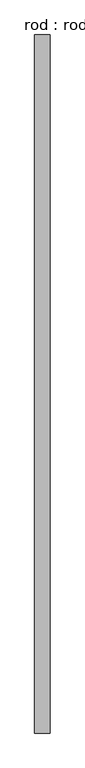
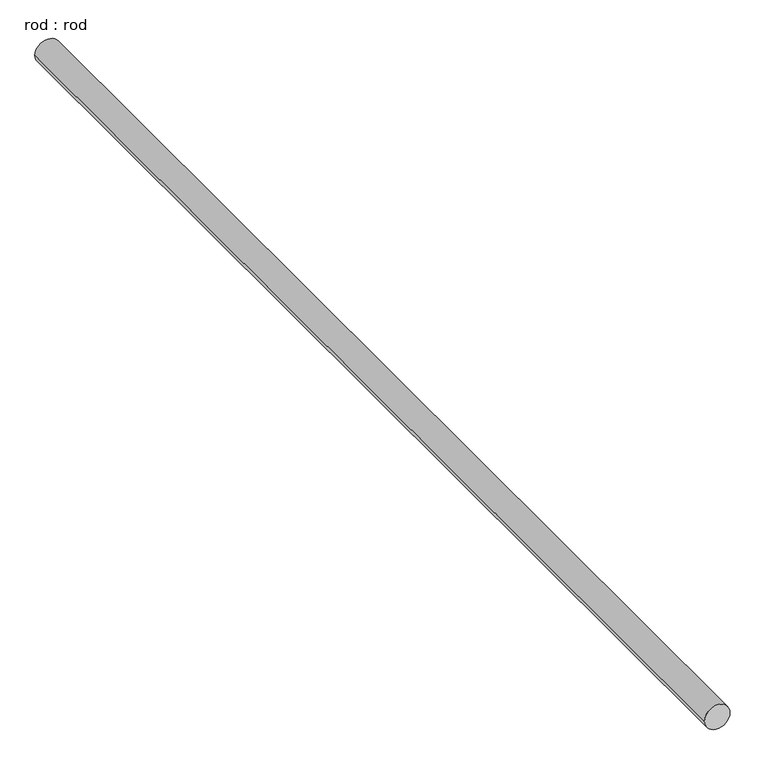
"""IFC4 building model written with IfcOpenShell, lengths in millimetres: proxy geometry, rod : rod."""

from ifc_helpers import new_model, si_unit, point, frame, frame_2d, origin, place, context, project, spatial, circle_curve, trimmed, segment, composite_curve, outline, extrude, source, transform, mapped, element, save


def rod_rod_ae1711a1(model_context):
    return source(origin(), model_context, "Body", "SweptSolid", [
        extrude(outline(composite_curve([segment(trimmed(circle_curve(frame_2d((0.0108462, 0.0)), 200.0), [point((0.0108462, 200.0))], [point((0.0108462, -200.0))], False, "CARTESIAN"), True, "CONTINUOUS"), segment(trimmed(circle_curve(frame_2d((0.0108462, 0.0)), 200.0), [point((0.0108462, -200.0))], [point((0.0108462, 200.0))], False, "CARTESIAN"), True, "CONTINUOUS")], self_intersect=False)), frame((0.0, -5029.4545229, 0.0), z_axis=(0.0, 1.0, 0.0), x_axis=(0.0, 0.0, 1.0)), (0.0, 0.0, 1.0), 18244.3662764),
    ])


if __name__ == "__main__":
    model = new_model("IFC4")
    model_context = context("Model", 3, world=origin())
    ifc_project = project(units=[si_unit("LENGTHUNIT", "METRE", prefix="MILLI")], contexts=[model_context])
    site = spatial("IfcSite", under=ifc_project)
    building = spatial("IfcBuilding", under=site)
    placement = place(None, origin())
    rod_rod_shape = rod_rod_ae1711a1(model_context)
    element("IfcBuildingElementProxy", 1, Name="rod : rod", ObjectType="rod : rod", at=placement, inside=building, context=model_context, shape_type="MappedRepresentation", body=[
        mapped(rod_rod_shape, transform((0.0, 0.0, 0.0), x_axis=(1.0, 0.0, 0.0), y_axis=(0.0, 1.0, 0.0), z_axis=(0.0, 0.0, 1.0))),
    ])
    save(model, "model.ifc")

# Revit data of these elements
# Type "rod : rod"
#   Default Elevation = 0
